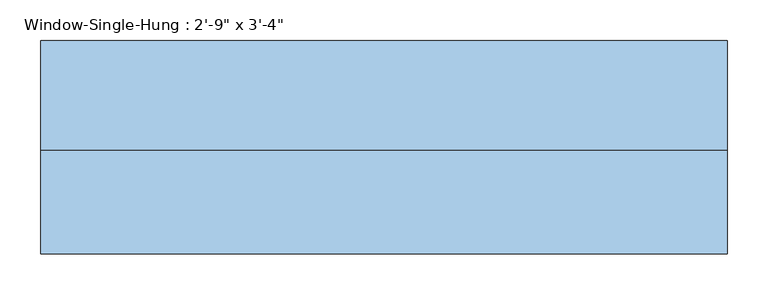
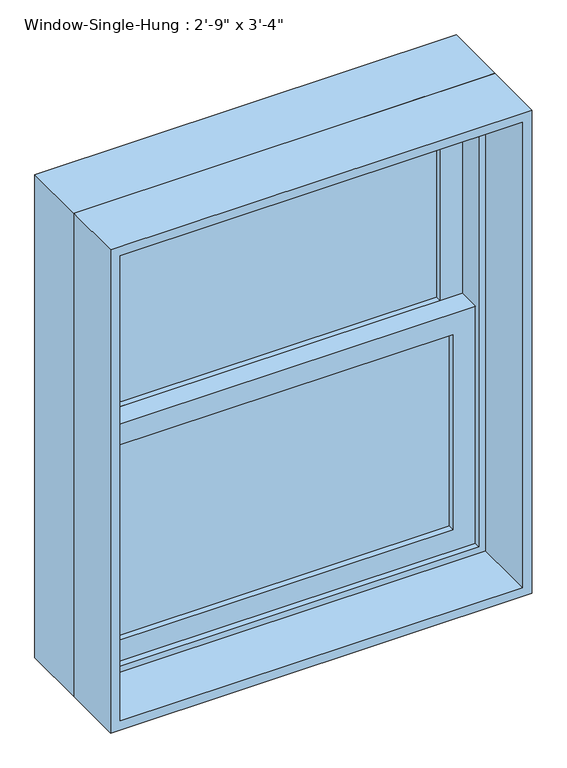
"""IFC4 building model written with IfcOpenShell, lengths in millimetres: window geometry."""

import ifcopenshell
import ifcopenshell.guid

model = None  # the IFC model being written
_history = None  # IfcOwnerHistory: only IFC2X3 demands one
_inside = {}  # id of a spatial element -> (the spatial element, [elements in it])
_under = {}  # id of a project, library or spatial element -> (it, [spatial elements below it])
_declared = {}  # id of a project -> (the project, [libraries it declares])
_typed = {}  # id of a type object -> (the type object, [elements of that type])
_made_of = {}  # id of a material, layer set ... -> (it, [elements and type objects made of it])


def new_model(schema):
    """Start an empty IFC model of exactly this schema.

    Asked for "IFC4X3", IfcOpenShell would pick the latest addendum, in which some entities
    have other attributes; the version numbers below select the first issue.
    IFC2X3 requires an IfcOwnerHistory on every rooted entity: one is made here for all.
    """
    global model, _history
    if schema == "IFC4X3":
        model = ifcopenshell.file(schema_version=(4, 3, 0, 0))
    else:
        model = ifcopenshell.file(schema=schema)
    _inside.clear()
    _under.clear()
    _declared.clear()
    _typed.clear()
    _made_of.clear()
    _history = None
    if model.schema == "IFC2X3":
        org = make("IfcOrganization", Name="unknown")
        user = make(
            "IfcPersonAndOrganization",
            ThePerson=make("IfcPerson", FamilyName="unknown"),
            TheOrganization=org,
        )
        app = make(
            "IfcApplication",
            ApplicationDeveloper=org,
            Version="unknown",
            ApplicationFullName="unknown",
            ApplicationIdentifier="unknown",
        )
        _history = make(
            "IfcOwnerHistory",
            OwningUser=user,
            OwningApplication=app,
            ChangeAction="ADDED",
            CreationDate=0,
        )
    return model


def make(cls, **values):
    """One entity of the class cls with the attributes given. An attribute that is None is left unset."""
    return model.create_entity(
        cls, **{name: value for name, value in values.items() if value is not None}
    )


def rooted(cls, **values):
    """An entity with a GlobalId (a new one), such as an element, a storey or a relation."""
    return make(cls, GlobalId=ifcopenshell.guid.new(), OwnerHistory=_history, **values)


def si_unit(unit_type, name, prefix=None):
    """IfcSIUnit, for example si_unit("LENGTHUNIT", "METRE", prefix="MILLI")."""
    return make("IfcSIUnit", UnitType=unit_type, Prefix=prefix, Name=name)


def assignment(units):
    """IfcUnitAssignment: the units of a project."""
    return None if units is None else make("IfcUnitAssignment", Units=units)


def point(xyz):
    """IfcCartesianPoint."""
    return None if xyz is None else make("IfcCartesianPoint", Coordinates=xyz)


def direction(xyz):
    """IfcDirection."""
    return None if xyz is None else make("IfcDirection", DirectionRatios=xyz)


def frame(location, z_axis=None, x_axis=None):
    """IfcAxis2Placement3D, a coordinate frame: its origin and axes. An axis left out is left unset."""
    return make(
        "IfcAxis2Placement3D",
        Location=point(location),
        Axis=direction(z_axis),
        RefDirection=direction(x_axis),
    )


def origin():
    """The frame at (0, 0, 0) with its axes left unset."""
    return frame((0.0, 0.0, 0.0))


def place(relative_to, where):
    """IfcLocalPlacement: puts the frame where relative to a parent placement (None: the world)."""
    return make(
        "IfcLocalPlacement", PlacementRelTo=relative_to, RelativePlacement=where
    )


def context(
    kind, dimensions, precision=None, world=None, true_north=None, identifier=None
):
    """IfcGeometricRepresentationContext, for example the 3D "Model" context."""
    return make(
        "IfcGeometricRepresentationContext",
        ContextIdentifier=identifier,
        ContextType=kind,
        CoordinateSpaceDimension=dimensions,
        Precision=precision,
        WorldCoordinateSystem=world,
        TrueNorth=true_north,
    )


def project(units=None, contexts=None):
    """IfcProject with its units and contexts."""
    return rooted(
        "IfcProject",
        Name="project",
        RepresentationContexts=contexts,
        UnitsInContext=assignment(units),
    )


def spatial(cls, under=None, at=None, **own):
    """A site, building, storey or space (cls), placed at a placement, below another one or the project."""
    s = rooted(cls, ObjectPlacement=at, **own)
    if under is not None:
        _under.setdefault(under.id(), (under, []))[1].append(s)
    return s


def polyline(points):
    """IfcPolyline through the points."""
    return make("IfcPolyline", Points=[point(p) for p in points])


def outline(outer, holes=None, kind="AREA"):
    """IfcArbitraryClosedProfileDef: a profile drawn as a closed curve; with holes, ...WithVoids."""
    if holes is None:
        return make("IfcArbitraryClosedProfileDef", ProfileType=kind, OuterCurve=outer)
    return make(
        "IfcArbitraryProfileDefWithVoids",
        ProfileType=kind,
        OuterCurve=outer,
        InnerCurves=holes,
    )


def extrude(swept, where, along, depth):
    """IfcExtrudedAreaSolid: the profile swept, set in the frame where, extruded along a direction by depth."""
    return make(
        "IfcExtrudedAreaSolid",
        SweptArea=swept,
        Position=where,
        ExtrudedDirection=direction(along),
        Depth=depth,
    )


def shape(context_of_items, identifier, shape_type, items):
    """IfcShapeRepresentation: the items that make up one representation, for example the "Body"."""
    return make(
        "IfcShapeRepresentation",
        ContextOfItems=context_of_items,
        RepresentationIdentifier=identifier,
        RepresentationType=shape_type,
        Items=items,
    )


def source(mapping_origin, context_of_items, identifier, shape_type, items):
    """IfcRepresentationMap: a shape defined once, which mapped items show again and again."""
    return make(
        "IfcRepresentationMap",
        MappingOrigin=mapping_origin,
        MappedRepresentation=shape(context_of_items, identifier, shape_type, items),
    )


def transform(
    local_origin,
    x_axis=None,
    y_axis=None,
    z_axis=None,
    scale=None,
    scale2=None,
    scale3=None,
    uniform=True,
):
    """IfcCartesianTransformationOperator3D, or its non-uniform kind. x_axis, y_axis, z_axis: its Axis1, 2, 3."""
    if uniform:
        return make(
            "IfcCartesianTransformationOperator3D",
            Axis1=direction(x_axis),
            Axis2=direction(y_axis),
            LocalOrigin=point(local_origin),
            Scale=scale,
            Axis3=direction(z_axis),
        )
    return make(
        "IfcCartesianTransformationOperator3DnonUniform",
        Axis1=direction(x_axis),
        Axis2=direction(y_axis),
        LocalOrigin=point(local_origin),
        Scale=scale,
        Axis3=direction(z_axis),
        Scale2=scale2,
        Scale3=scale3,
    )


def mapped(mapping_source, mapping_target):
    """IfcMappedItem: shows the shape of a source again, moved by a transform."""
    return make(
        "IfcMappedItem", MappingSource=mapping_source, MappingTarget=mapping_target
    )


def made_of(thing, what):
    """Note that an element or type object is made of a material, layer set ...; save() writes the relation."""
    if what is not None:
        _made_of.setdefault(what.id(), (what, []))[1].append(thing)
    return thing


def element(
    cls,
    number,
    at=None,
    inside=None,
    cuts=None,
    type_object=None,
    material=None,
    context=None,
    identifier="Body",
    shape_type=None,
    held_by="IfcProductDefinitionShape",
    body=None,
    shapes=None,
    **own,
):
    """One element of the class cls, such as IfcWall. Its Tag is "e" and its number.

    at: its placement. inside: the storey or other place that contains it. cuts: it is an
    opening in that element (IfcRelVoidsElement). A single representation is given by context,
    identifier, shape_type and body (its items); several are given by shapes. held_by: the class
    of the entity that holds the representations. save() writes the other relations.
    """
    e = rooted(cls, Tag="e%d" % number, ObjectPlacement=at, **own)
    if body is not None:
        shapes = [shape(context, identifier, shape_type, body)]
    if shapes is not None:
        e.Representation = make(held_by, Representations=shapes)
    if inside is not None:
        _inside.setdefault(inside.id(), (inside, []))[1].append(e)
    if cuts is not None:
        rooted(
            "IfcRelVoidsElement", RelatingBuildingElement=cuts, RelatedOpeningElement=e
        )
    if type_object is not None:
        _typed.setdefault(type_object.id(), (type_object, []))[1].append(e)
    return made_of(e, material)


def aggregate(whole, parts):
    """IfcRelAggregates: a whole, such as a stair, and the parts it consists of."""
    return rooted("IfcRelAggregates", RelatingObject=whole, RelatedObjects=parts)


def save(model, path):
    """Write the relations noted so far, then the file.

    IfcRelAggregates (storeys below a building ...), IfcRelContainedInSpatialStructure (elements
    in a storey), IfcRelDefinesByType, IfcRelAssociatesMaterial and IfcRelDeclares: one each for
    every whole, place, type object, material and project.
    """
    for whole, parts in _under.values():
        aggregate(whole, parts)
    for where, things in _inside.values():
        rooted(
            "IfcRelContainedInSpatialStructure",
            RelatedElements=things,
            RelatingStructure=where,
        )
    for kind, things in _typed.values():
        rooted("IfcRelDefinesByType", RelatedObjects=things, RelatingType=kind)
    for what, things in _made_of.values():
        rooted("IfcRelAssociatesMaterial", RelatedObjects=things, RelatingMaterial=what)
    for by, libraries in _declared.values():
        rooted("IfcRelDeclares", RelatingContext=by, RelatedDefinitions=libraries)
    model.write(path)


def window_aaa0cff3(model_context):
    return source(origin(), model_context, "Body", "SweptSolid", [
        extrude(outline(polyline([(342.9, 50.8), (342.9, 44.45), (-342.9, 44.45), (-342.9, 50.8), (342.9, 50.8)])), frame((0.0, 0.0, 990.6), z_axis=(0.0, 0.0, 1.0), x_axis=(1.0, 0.0, 0.0)), (0.0, 0.0, 1.0), 409.575),
        extrude(outline(polyline([(-342.9, 38.1), (342.9, 38.1), (342.9, 31.75), (-342.9, 31.75), (-342.9, 38.1)])), frame((0.0, 0.0, 990.6), z_axis=(0.0, 0.0, 1.0), x_axis=(1.0, 0.0, 0.0)), (0.0, 0.0, 1.0), 409.575),
        extrude(outline(polyline([(342.9, 95.25), (342.9, 88.9), (-342.9, 88.9), (-342.9, 95.25), (342.9, 95.25)])), frame((0.0, 0.0, 1444.625), z_axis=(0.0, 0.0, 1.0), x_axis=(1.0, 0.0, 0.0)), (0.0, 0.0, 1.0), 409.575),
        extrude(outline(polyline([(-342.9, 82.55), (342.9, 82.55), (342.9, 76.2), (-342.9, 76.2), (-342.9, 82.55)])), frame((0.0, 0.0, 1444.625), z_axis=(0.0, 0.0, 1.0), x_axis=(1.0, 0.0, 0.0)), (0.0, 0.0, 1.0), 409.575),
        extrude(outline(polyline([(1444.625, -387.35), (946.15, -387.35), (946.15, 387.35), (1444.625, 387.35), (1444.625, -387.35)]), holes=[polyline([(1400.175, 342.9), (990.6, 342.9), (990.6, -342.9), (1400.175, -342.9), (1400.175, 342.9)])]), frame((0.0, 19.05, 0.0), z_axis=(0.0, 1.0, 0.0), x_axis=(0.0, 0.0, 1.0)), (0.0, 0.0, 1.0), 44.45),
        extrude(outline(polyline([(1898.65, -387.35), (1400.175, -387.35), (1400.175, 387.35), (1898.65, 387.35), (1898.65, -387.35)]), holes=[polyline([(1854.2, 342.9), (1444.625, 342.9), (1444.625, -342.9), (1854.2, -342.9), (1854.2, 342.9)])]), frame((0.0, 63.5, 0.0), z_axis=(0.0, 1.0, 0.0), x_axis=(0.0, 0.0, 1.0)), (0.0, 0.0, 1.0), 44.45),
        extrude(outline(polyline([(1930.4, -419.1), (914.4, -419.1), (914.4, 419.1), (1930.4, 419.1), (1930.4, -419.1)]), holes=[polyline([(1898.65, 387.35), (946.15, 387.35), (946.15, -387.35), (1898.65, -387.35), (1898.65, 387.35)])]), frame((0.0, 6.35, 0.0), z_axis=(0.0, 1.0, 0.0), x_axis=(0.0, 0.0, 1.0)), (0.0, 0.0, 1.0), 133.35),
        extrude(outline(polyline([(1930.4, 419.1), (1930.4, -419.1), (914.4, -419.1), (914.4, 419.1), (1930.4, 419.1)]), holes=[polyline([(1911.35, 400.05), (933.45, 400.05), (933.45, -400.05), (1911.35, -400.05), (1911.35, 400.05)])]), frame((0.0, -120.65, 0.0), z_axis=(0.0, 1.0, 0.0), x_axis=(0.0, 0.0, 1.0)), (0.0, 0.0, 1.0), 127.0),
    ])


if __name__ == "__main__":
    model = new_model("IFC4")
    model_context = context("Model", 3, world=origin())
    ifc_project = project(units=[si_unit("LENGTHUNIT", "METRE", prefix="MILLI")], contexts=[model_context])
    site = spatial("IfcSite", under=ifc_project)
    building = spatial("IfcBuilding", under=site)
    placement = place(None, origin())
    window_shape = window_aaa0cff3(model_context)
    element("IfcWindow", 1, ObjectType="Window-Single-Hung : 2'-9\" x 3'-4\"", at=placement, inside=building, context=model_context, shape_type="MappedRepresentation", body=[
        mapped(window_shape, transform((0.0, 0.0, 0.0), x_axis=(1.0, 0.0, 0.0), y_axis=(0.0, 1.0, 0.0), z_axis=(0.0, 0.0, 1.0))),
    ])
    save(model, "model.ifc")

# Revit data of these elements
# Type "Window-Single-Hung : 2'-9\" x 3'-4\""
#   Type Mark = "22"
#   Fire Rating = "0.5h"
#   Construction Type Id = "DG-DR"
#   Assembly Code = "B2020100"
#   Analytic Construction = "Double glazing - domestic"
#   Wall Thickness [instance default] = 0' - 6"
#   Window Inset [instance default] = 0' - 0"
#   Visual Light Transmittance = 0.81
#   Thermal Resistance (R) = 0.319569 (m²·K)/W
#   Solar Heat Gain Coefficient = 0.76
#   Muntin Width = 2' - 3"
#   Muntin Height = 1' - 4 1/8"
#   Interior Wall Closure [instance default] = 0' - 1 1/2"
#   Rough Width = 2' - 9 1/2"
#   Rough Height = 3' - 4 1/2"
#   Frame Extension [instance default] = 0' - 1 1/4"
#   Exterior Wall Closure [instance default] = 0' - 0 1/2"
#   Extension Jamb [instance default] = 0' - 1 1/2"
#   Heat Transfer Coefficient (U) = 3.12929 W/(m²·K)
#   Height = 3' - 4"
#   Width = 2' - 9"
#   Top Muntin Visibility = yes
#   Indicator Visibility [instance default] = yes
#   Extension Jamb Visibility [instance default] = yes
#   Interior Trim Visibility [instance default] = yes
#   Exterior Trim Visibility [instance default] = yes
#   Bottom Muntin Visibility = yes
#   Muntin Pattern = Muntin Pattern_2x2 : Muntin Pattern_2x2
#   Interior Trim Material = Wood - Stained
#   Interior Trim = Trim-Window-Interior-Flat : Picture Frame
#   Exterior Trim Material = Clad - White
#   Exterior Trim = Trim-Window-Exterior-Flat : with Sill
#   Glass Panel Material = Glass
#   Exterior Frame Material = Clad - White
#   Interior Frame Material = Wood - Stained
#   Wall Closure = (empty or 0)
# Element 1 (IfcWindow, "Window-Single-Hung : 2'-9\" x 3'-4\"")
#   Wall Thickness = 0' - 9 1/2"
#   Extension Jamb = 0' - 5"
#   Materials on its faces: "Wood - Stained", "Glass", "Clad - White"
# Materials
#   "Wood - Stained": class "Wood", colour RGB 224 178 126, transparency 0, Cost = 0
#   "Clad - White": class "Wood", colour RGB 242 242 238, transparency 0, Cost = 0
#   "Glass": class "Glass", colour RGB 218 227 224, transparency 0.85, Description = "Soda Lime Glass", Cost = 0
